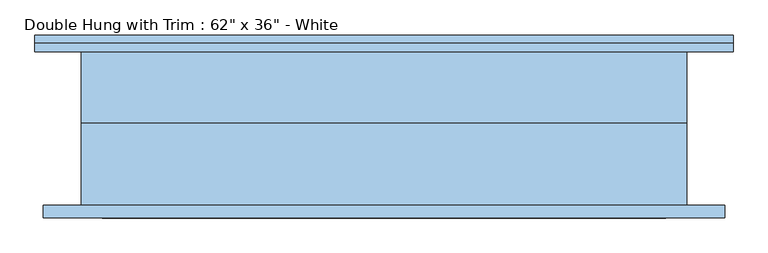
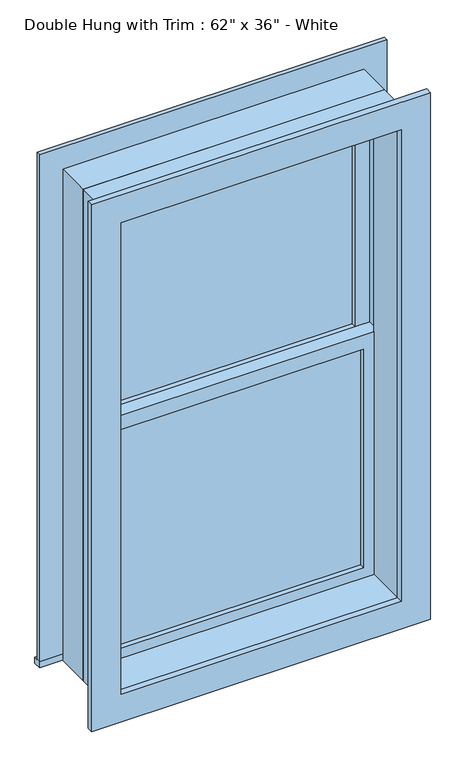
"""IFC4 building model written with IfcOpenShell, lengths in millimetres: window geometry."""

from ifc_helpers import new_model, si_unit, frame, origin, place, context, project, spatial, polyline, outline, extrude, source, transform, mapped, element, save


def window_5270e79a(model_context):
    return source(origin(), model_context, "Body", "SweptSolid", [
        extrude(outline(polyline([(-393.7, 36.5125008), (393.7, 36.5125008), (393.7, 23.8125008), (-393.7, 23.8125008), (-393.7, 36.5125008)])), frame((0.0, 0.0, 571.5), z_axis=(0.0, 0.0, 1.0), x_axis=(1.0, 0.0, 0.0)), (0.0, 0.0, 1.0), 701.675),
        extrude(outline(polyline([(1317.625, -438.15), (527.05, -438.15), (527.05, 438.15), (1317.625, 438.15), (1317.625, -438.15)]), holes=[polyline([(1273.175, -393.7), (1273.175, 393.7), (571.5, 393.7), (571.5, -393.7), (1273.175, -393.7)])]), frame((0.0, 7.9375008, 0.0), z_axis=(0.0, 1.0, 0.0), x_axis=(0.0, 0.0, 1.0)), (0.0, 0.0, 1.0), 44.45),
        extrude(outline(polyline([(-527.05, 141.2875008), (527.05, 141.2875008), (527.05, 115.8875008), (-527.05, 115.8875008), (-527.05, 141.2875008)])), frame((0.0, 0.0, 508.0), z_axis=(0.0, 0.0, 1.0), x_axis=(1.0, 0.0, 0.0)), (0.0, 0.0, 1.0), 19.05),
        extrude(outline(polyline([(2063.75, -438.15), (2063.75, 438.15), (527.05, 438.15), (527.05, 527.05), (2152.65, 527.05), (2152.65, -527.05), (527.05, -527.05), (527.05, -438.15), (2063.75, -438.15)])), frame((0.0, 115.8875008, 0.0), z_axis=(0.0, 1.0, 0.0), x_axis=(0.0, 0.0, 1.0)), (0.0, 0.0, 1.0), 12.7),
        extrude(outline(polyline([(2139.95, 514.35), (2139.95, -514.35), (450.85, -514.35), (450.85, 514.35), (2139.95, 514.35)]), holes=[polyline([(2051.05, 425.45), (539.75, 425.45), (539.75, -425.45), (2051.05, -425.45), (2051.05, 425.45)])]), frame((0.0, -134.9375008, 0.0), z_axis=(0.0, 1.0, 0.0), x_axis=(0.0, 0.0, 1.0)), (0.0, 0.0, 1.0), 19.05),
        extrude(outline(polyline([(393.7, 68.2625008), (-393.7, 68.2625008), (-393.7, 80.9625008), (393.7, 80.9625008), (393.7, 68.2625008)])), frame((0.0, 0.0, 1317.625), z_axis=(0.0, 0.0, 1.0), x_axis=(1.0, 0.0, 0.0)), (0.0, 0.0, 1.0), 701.675),
        extrude(outline(polyline([(2063.75, -438.15), (1273.175, -438.15), (1273.175, 438.15), (2063.75, 438.15), (2063.75, -438.15)]), holes=[polyline([(2019.3, -393.7), (2019.3, 393.7), (1317.625, 393.7), (1317.625, -393.7), (2019.3, -393.7)])]), frame((0.0, 52.3875008, 0.0), z_axis=(0.0, 1.0, 0.0), x_axis=(0.0, 0.0, 1.0)), (0.0, 0.0, 1.0), 44.45),
        extrude(outline(polyline([(2082.8, -457.2), (508.0, -457.2), (508.0, 457.2), (2082.8, 457.2), (2082.8, -457.2)]), holes=[polyline([(2051.05, -425.45), (2051.05, 425.45), (539.75, 425.45), (539.75, -425.45), (2051.05, -425.45)])]), frame((0.0, -115.8875008, 0.0), z_axis=(0.0, 1.0, 0.0), x_axis=(0.0, 0.0, 1.0)), (0.0, 0.0, 1.0), 123.8250015),
        extrude(outline(polyline([(2082.8, 457.2), (2082.8, -457.2), (508.0, -457.2), (508.0, 457.2), (2082.8, 457.2)]), holes=[polyline([(2063.75, 438.15), (527.05, 438.15), (527.05, -438.15), (2063.75, -438.15), (2063.75, 438.15)])]), frame((0.0, 7.9375008, 0.0), z_axis=(0.0, 1.0, 0.0), x_axis=(0.0, 0.0, 1.0)), (0.0, 0.0, 1.0), 107.95),
    ])


if __name__ == "__main__":
    model = new_model("IFC4")
    model_context = context("Model", 3, world=origin())
    ifc_project = project(units=[si_unit("LENGTHUNIT", "METRE", prefix="MILLI")], contexts=[model_context])
    site = spatial("IfcSite", under=ifc_project)
    building = spatial("IfcBuilding", under=site)
    placement = place(None, origin())
    window_shape = window_5270e79a(model_context)
    element("IfcWindow", 1, ObjectType="Double Hung with Trim : 62\" x 36\" - White", at=placement, inside=building, context=model_context, shape_type="MappedRepresentation", body=[
        mapped(window_shape, transform((0.0, 0.0, 0.0), x_axis=(1.0, 0.0, 0.0), y_axis=(0.0, 1.0, 0.0), z_axis=(0.0, 0.0, 1.0))),
    ])
    save(model, "model.ifc")

# Revit data of these elements
# Type "Double Hung with Trim : 62\" x 36\" - White"
#   Type Mark = "81"
#   Construction Type Id = "GSP4R"
#   Assembly Code = "B2020100"
#   Analytic Construction = "1/8 in Pilkington single glazing"
#   Visual Light Transmittance = 0.9
#   Solar Heat Gain Coefficient = 0.78
#   Heat Transfer Coefficient (U) = 3.6886 W/(m²·K)
#   Height = 5' - 2"
#   Default Sill Height = 1' - 8"
#   Trim Projection - Ext. = 0' - 0 1/2"
#   Trim Projection - Int. = 0' - 0 3/4"
#   Trim Width - Exterior = 0' - 3 1/2"
#   Trim Width - Interior = 0' - 3 1/2"
#   Width = 3' - 0"
#   Window Inset = 0' - 0 3/4"
#   Glass Pane Material = Glass
#   Sash Material = Sash - White
#   Trim Exterior Material = Trim - White
#   Trim Interior Material = Trim - White
#   Wall Closure = (empty or 0)
# Element 1 (IfcWindow, "Double Hung with Trim : 62\" x 36\" - White")
#   Materials on its faces: "Sash - White", "Trim - White", "Glass"
# Materials
#   "Glass": class "Glass", colour RGB 0 128 192, transparency 0.75, Description = "Soda Lime Glass", Cost = 0
#   "Sash - White": class "Wood", colour RGB 255 255 255, transparency 0, Cost = 0
#   "Trim - White": class "Wood", colour RGB 255 255 255, transparency 0, Cost = 0
